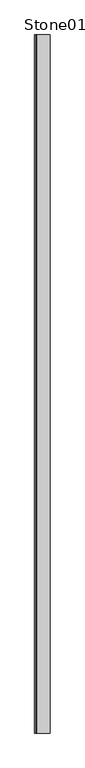
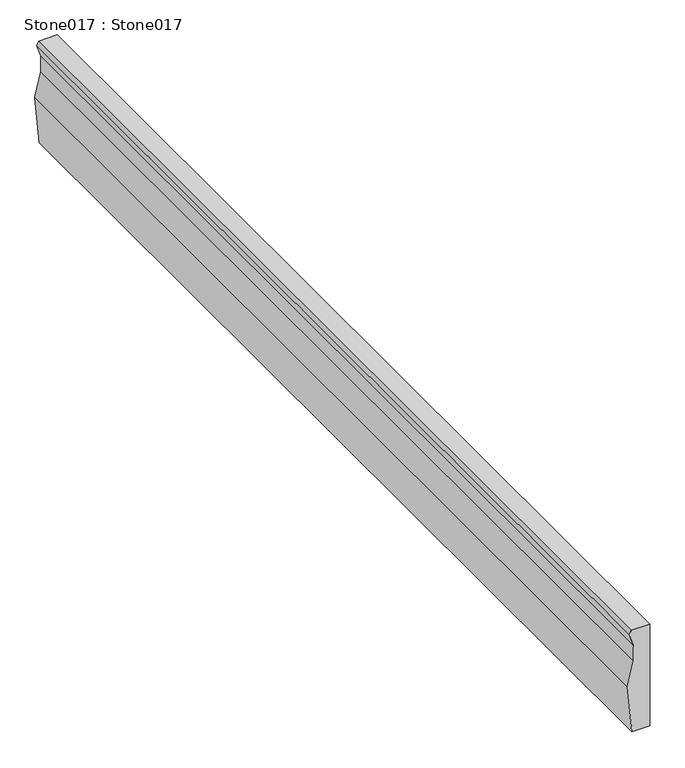
"""IFC4 building model written with IfcOpenShell, lengths in millimetres: proxy geometry, Stone017 : Stone017."""

from ifc_helpers import new_model, si_unit, frame, origin, place, context, project, spatial, polyline, outline, extrude, source, transform, mapped, element, save


def stone017_stone017_f5c83055(model_context):
    return source(origin(), model_context, "Body", "SweptSolid", [
        extrude(outline(polyline([(33394.2430685, -10302.7509766), (33385.90625, -10305.9892578), (33362.4765625, -10298.8007813), (33330.0664062, -10298.3115234), (33280.7148437, -10309.8115234), (33185.140625, -10301.6737014), (33185.140625, -10266.1494141), (33394.2430685, -10266.1494141), (33394.2430685, -10302.7509766)])), frame((0.0, 7982.1531721, 0.0), z_axis=(0.0, 1.0, 0.0), x_axis=(0.0, 0.0, 1.0)), (0.0, 0.0, 1.0), 2000.0),
    ])


if __name__ == "__main__":
    model = new_model("IFC4")
    model_context = context("Model", 3, world=origin())
    ifc_project = project(units=[si_unit("LENGTHUNIT", "METRE", prefix="MILLI")], contexts=[model_context])
    site = spatial("IfcSite", under=ifc_project)
    building = spatial("IfcBuilding", under=site)
    placement = place(None, origin())
    stone017_stone017_shape = stone017_stone017_f5c83055(model_context)
    element("IfcBuildingElementProxy", 1, Name="Stone017 : Stone017", ObjectType="Stone017 : Stone017", at=placement, inside=building, context=model_context, shape_type="MappedRepresentation", body=[
        mapped(stone017_stone017_shape, transform((0.0, 0.0, 0.0), x_axis=(1.0, 0.0, 0.0), y_axis=(0.0, 1.0, 0.0), z_axis=(0.0, 0.0, 1.0))),
    ])
    save(model, "model.ifc")

# Revit data of these elements
# Type "Stone017 : Stone017"
#   NameOverride = "Stone017"
# Element 1 (IfcBuildingElementProxy, "Stone017 : Stone017")
#   Materials on its faces: "SPLIT FACE STONE"
# Materials
#   "SPLIT FACE STONE": class "Unassigned", colour RGB 205 195 181, transparency 0, Cost = 0
